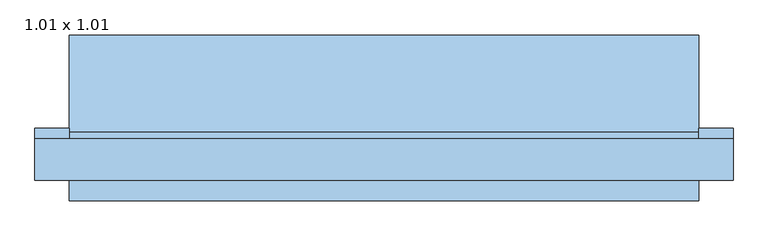
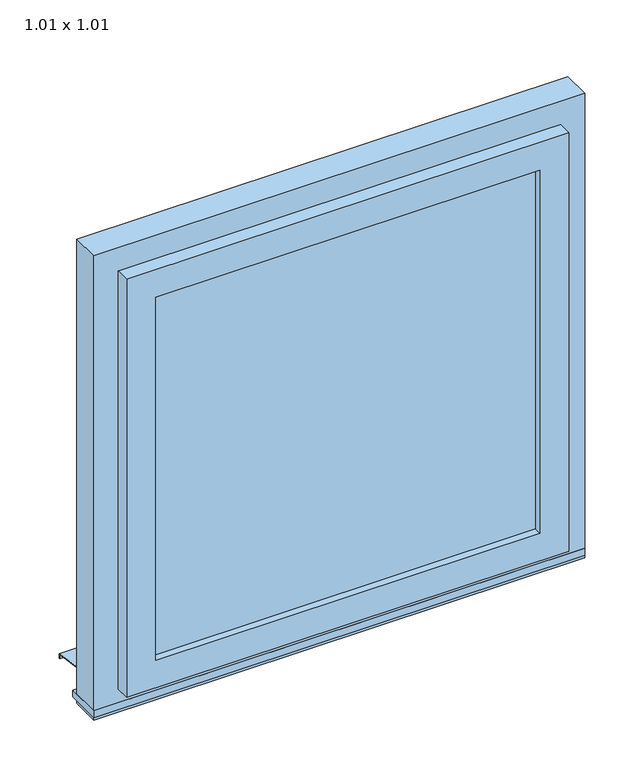
"""IFC4 building model written with IfcOpenShell, lengths in millimetres: window geometry, Fenster 1-flg - Anschlag : 1.01 x 1.01."""

from ifc_helpers import new_model, si_unit, frame, origin, place, context, project, spatial, polyline, outline, extrude, faceted_brep, source, transform, mapped, element, save


def window_1_01_x_1_01_37b9fed5(model_context):
    return source(origin(), model_context, "Body", "SolidModel", [
        extrude(outline(polyline([(-525.0, -142.5), (-525.0, -67.5), (-475.0, -67.5), (-475.0, -82.5), (435.0, -82.5), (435.0, -67.5), (485.0, -67.5), (485.0, -142.5), (-525.0, -142.5)])), frame((0.0, 0.0, 1005.0), z_axis=(0.0, 0.0, 1.0), x_axis=(1.0, 0.0, 0.0)), (0.0, 0.0, 1.0), 15.0),
        extrude(outline(polyline([(375.0, -157.5), (-415.0, -157.5), (-415.0, -127.5), (375.0, -127.5), (375.0, -157.5)])), frame((0.0, 0.0, 1110.0), z_axis=(0.0, 0.0, 1.0), x_axis=(1.0, 0.0, 0.0)), (0.0, 0.0, 1.0), 790.0),
        extrude(outline(polyline([(-72.4778457, 1020.0), (67.5, 1000.0), (67.5, 990.0), (65.5, 990.0), (65.5, 998.3604634), (-72.6759277, 1018.0), (-82.5, 1018.0), (-82.5, 1020.0), (-72.4778457, 1020.0)])), frame((-475.0, 0.0, 0.0), z_axis=(1.0, 0.0, 0.0), x_axis=(0.0, 1.0, 0.0)), (0.0, 0.0, 1.0), 910.0),
        extrude(outline(polyline([(2010.0, 485.0), (2010.0, -525.0), (1000.0, -525.0), (1000.0, 485.0), (2010.0, 485.0)]), holes=[polyline([(1930.0, 405.0), (1080.0, 405.0), (1080.0, -445.0), (1930.0, -445.0), (1930.0, 405.0)])]), frame((0.0, -142.5, 0.0), z_axis=(0.0, 1.0, 0.0), x_axis=(0.0, 0.0, 1.0)), (0.0, 0.0, 1.0), 60.0),
        faceted_brep([(435.0, -142.5, 1960.0), (435.0, -172.5, 1960.0), (435.0, -172.5, 1050.0), (435.0, -142.5, 1050.0), (-475.0, -172.5, 1960.0), (-475.0, -172.5, 1050.0), (375.0, -172.5, 1110.0), (-415.0, -172.5, 1110.0), (-415.0, -172.5, 1900.0), (375.0, -172.5, 1900.0), (-475.0, -142.5, 1050.0), (-475.0, -142.5, 1960.0), (405.0, -142.5, 1930.0), (-445.0, -142.5, 1930.0), (-445.0, -142.5, 1080.0), (405.0, -142.5, 1080.0), (405.0, -112.5, 1930.0), (405.0, -112.5, 1080.0), (-445.0, -112.5, 1080.0), (-445.0, -112.5, 1930.0), (375.0, -112.5, 1900.0), (-415.0, -112.5, 1900.0), (-415.0, -112.5, 1110.0), (375.0, -112.5, 1110.0)], [[[0, 1, 2, 3]], [[1, 4, 5, 2], [6, 7, 8, 9]], [[3, 2, 5, 10]], [[3, 10, 11, 0], [12, 13, 14, 15]], [[16, 12, 15, 17]], [[17, 15, 14, 18]], [[17, 18, 19, 16], [20, 21, 22, 23]], [[9, 20, 23, 6]], [[6, 23, 22, 7]], [[10, 5, 4, 11]], [[18, 14, 13, 19]], [[7, 22, 21, 8]], [[11, 4, 1, 0]], [[19, 13, 12, 16]], [[8, 21, 20, 9]]]),
    ])


if __name__ == "__main__":
    model = new_model("IFC4")
    model_context = context("Model", 3, world=origin())
    ifc_project = project(units=[si_unit("LENGTHUNIT", "METRE", prefix="MILLI")], contexts=[model_context])
    site = spatial("IfcSite", under=ifc_project)
    building = spatial("IfcBuilding", under=site)
    placement = place(None, origin())
    window_1_01_x_1_01_shape = window_1_01_x_1_01_37b9fed5(model_context)
    element("IfcWindow", 1, ObjectType="Fenster 1-flg - Anschlag : 1.01 x 1.01", at=placement, inside=building, context=model_context, shape_type="MappedRepresentation", body=[
        mapped(window_1_01_x_1_01_shape, transform((0.0, 0.0, 0.0), x_axis=(1.0, 0.0, 0.0), y_axis=(0.0, 1.0, 0.0), z_axis=(0.0, 0.0, 1.0))),
    ])
    save(model, "model.ifc")

# Revit data of these elements
# Type "Fenster 1-flg - Anschlag : 1.01 x 1.01"
#   Type Mark = "47"
#   Operation = "SinglePanel"
#   Keynote = "16.05.01"
#   Construction Type Id = "GSP4R"
#   Analytic Construction = "1/8 Zoll Pilkington-Verglasung einfach"
#   Visual Light Transmittance = 0.9
#   Thermal Resistance (R) = 0.1491 (m²·K)/W
#   Solar Heat Gain Coefficient = 0.86
#   Anschlagsbreite seitlich = 0.050 m
#   Rough Width = 1.010 m
#   Rough Height = 1.010 m
#   Heat Transfer Coefficient (U) = 6.7069 W/(m²·K)
#   Rahmentiefe = 0.060 m
#   Rahmenhöhe unten = 0.080 m
#   Höhe oberer  Rahmen = 0.080 m
#   Rahmenbreite = 0.080 m
#   Height = 1.010 m
#   Tiefe Flügel = 0.060 m
#   Flügelbreite = 0.060 m
#   Einbautiefe (von außen) [instance default] = 0.120 m
#   Width = 1.010 m
#   Anschlagsbreite oben = 0.050 m
#   Klappflügel [instance default] = no
#   Öffnungsrichtung oben [instance default] = yes
#   Öffnungsrichtung in Draufsicht anzeigen [instance default] = no
#   Drehflügel 1 [instance default] = yes
#   Bild [instance default] = none
#   Glas [instance default] = none
#   Fensterflügel [instance default] = none
#   Innere Fensterbank [instance default] = none
#   Äußere Fensterbank [instance default] = none
#   Wall Closure = (empty or 0)
# Element 1 (IfcWindow, "Fenster 1-flg - Anschlag : 1.01 x 1.01")
#   Materials on its faces: "Kunststoff - Weiß", "Holz - Birke", "Glas"
# Materials
#   "Kunststoff - Weiß": class "Kunststoff", colour RGB 249 249 249, transparency 0, Cost = 0
#   "Holz - Birke": class "Holz", colour RGB 213 164 103, transparency 0, Cost = 0
#   "Glas": class "Glas", colour RGB 0 0 255, transparency 0.75, Comments = "Render-Darstellung nicht aktualisiert ", Cost = 0
